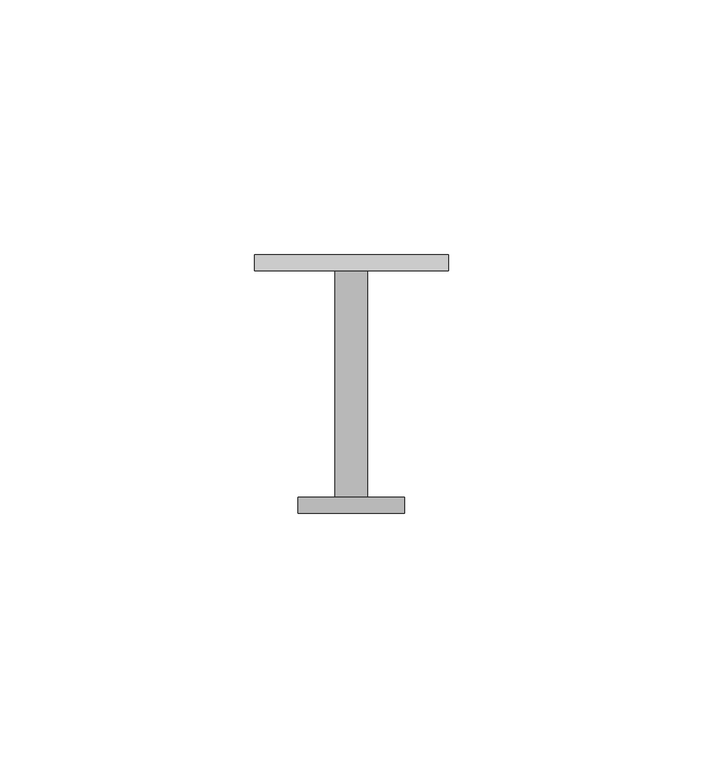
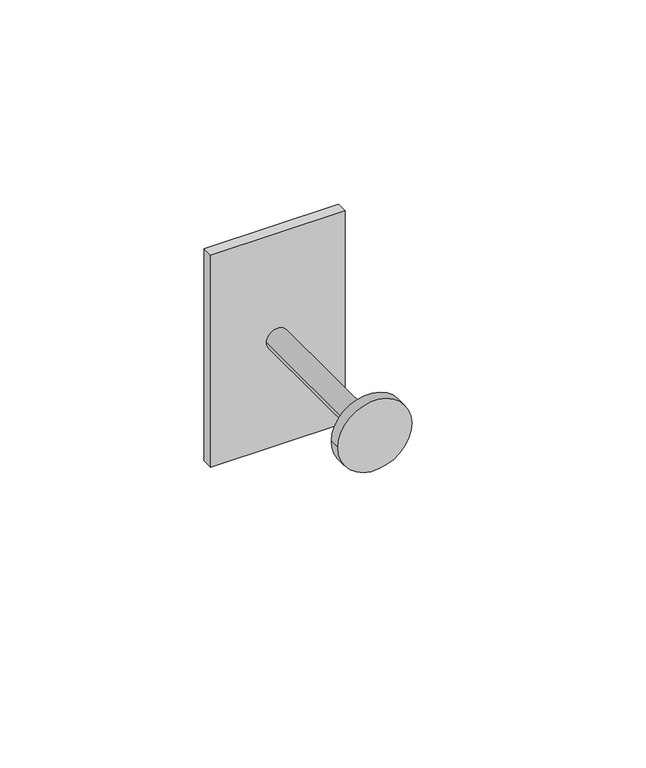
"""IFC4 building model written with IfcOpenShell, lengths in millimetres: proxy geometry, Hook, Garment and Towel - NON-COLLECTUS : -."""

from ifc_helpers import new_model, si_unit, point, frame, frame_2d, origin, origin_with_axes, place, context, project, spatial, polyline, circle_curve, trimmed, segment, composite_curve, outline, extrude, source, transform, mapped, element, save


def specialty_equipment_a72cc0be(model_context):
    return source(origin(), model_context, "Body", "SweptSolid", [
        extrude(outline(composite_curve([segment(trimmed(circle_curve(frame_2d((31.75, 19.05)), 10.4588235), [point((31.75, 29.5088235))], [point((31.75, 8.5911765))], False, "CARTESIAN"), True, "CONTINUOUS"), segment(trimmed(circle_curve(frame_2d((31.75, 19.05)), 10.4588235), [point((31.75, 8.5911765))], [point((31.75, 29.5088235))], False, "CARTESIAN"), True, "CONTINUOUS")], self_intersect=False)), frame((0.0, -50.8, 0.0), z_axis=(0.0, 1.0, 0.0), x_axis=(0.0, 0.0, 1.0)), (0.0, 0.0, 1.0), 3.175),
        extrude(outline(composite_curve([segment(trimmed(circle_curve(frame_2d((31.75, 19.05)), 3.175), [point((31.75, 22.225))], [point((31.75, 15.875))], False, "CARTESIAN"), True, "CONTINUOUS"), segment(trimmed(circle_curve(frame_2d((31.75, 19.05)), 3.175), [point((31.75, 15.875))], [point((31.75, 22.225))], False, "CARTESIAN"), True, "CONTINUOUS")], self_intersect=False)), frame((0.0, -47.625, 0.0), z_axis=(0.0, 1.0, 0.0), x_axis=(0.0, 0.0, 1.0)), (0.0, 0.0, 1.0), 44.45),
        extrude(outline(polyline([(38.1, -3.175), (0.0, -3.175), (0.0, 0.0), (38.1, 0.0), (38.1, -3.175)])), origin_with_axes(), (0.0, 0.0, 1.0), 63.5),
    ])


if __name__ == "__main__":
    model = new_model("IFC4")
    model_context = context("Model", 3, world=origin())
    ifc_project = project(units=[si_unit("LENGTHUNIT", "METRE", prefix="MILLI")], contexts=[model_context])
    site = spatial("IfcSite", under=ifc_project)
    building = spatial("IfcBuilding", under=site)
    placement = place(None, origin())
    specialty_equipment_shape = specialty_equipment_a72cc0be(model_context)
    element("IfcBuildingElementProxy", 1, Name="Hook, Garment and Towel - NON-COLLECTUS : -", ObjectType="Hook, Garment and Towel - NON-COLLECTUS : -", at=placement, inside=building, context=model_context, shape_type="MappedRepresentation", body=[
        mapped(specialty_equipment_shape, transform((0.0, 0.0, 0.0), x_axis=(1.0, 0.0, 0.0), y_axis=(0.0, 1.0, 0.0), z_axis=(0.0, 0.0, 1.0))),
    ])
    save(model, "model.ifc")

# Revit data of these elements
# Type "Hook, Garment and Towel - NON-COLLECTUS : -"
#   External ID [instance default] = ""
#   Width = 38.1 mm
#   Height = 63.5 mm
#   Depth = 50.8 mm
#   Material = Light Grey
#   Default Elevation = 0
# Element 1 (IfcBuildingElementProxy, "Hook, Garment and Towel - NON-COLLECTUS : -")
#   Materials on its faces: "Light Grey"
# Materials
#   "Light Grey": class "Generic", colour RGB 215 215 215, transparency 0, Cost = 0
